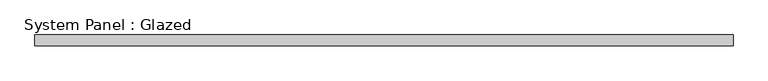
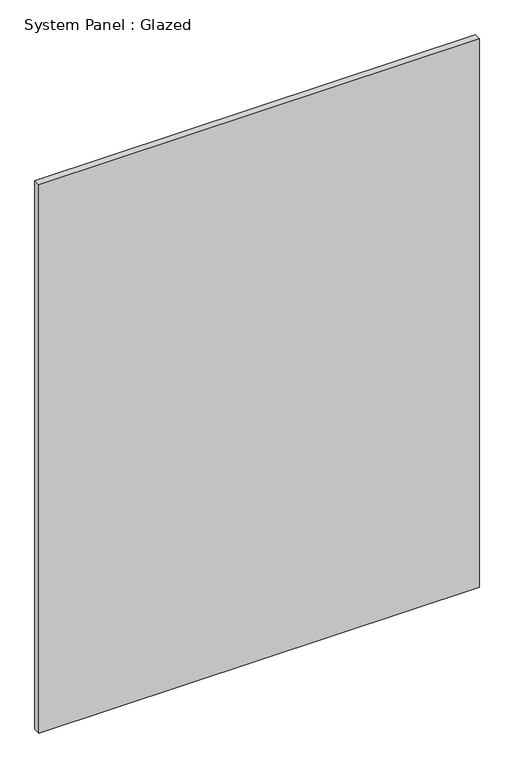
"""IFC4 building model written with IfcOpenShell, lengths in millimetres: plate geometry, System Panel : Glazed."""

import ifcopenshell
import ifcopenshell.guid

model = None  # the IFC model being written
_history = None  # IfcOwnerHistory: only IFC2X3 demands one
_inside = {}  # id of a spatial element -> (the spatial element, [elements in it])
_under = {}  # id of a project, library or spatial element -> (it, [spatial elements below it])
_declared = {}  # id of a project -> (the project, [libraries it declares])
_typed = {}  # id of a type object -> (the type object, [elements of that type])
_made_of = {}  # id of a material, layer set ... -> (it, [elements and type objects made of it])


def new_model(schema):
    """Start an empty IFC model of exactly this schema.

    Asked for "IFC4X3", IfcOpenShell would pick the latest addendum, in which some entities
    have other attributes; the version numbers below select the first issue.
    IFC2X3 requires an IfcOwnerHistory on every rooted entity: one is made here for all.
    """
    global model, _history
    if schema == "IFC4X3":
        model = ifcopenshell.file(schema_version=(4, 3, 0, 0))
    else:
        model = ifcopenshell.file(schema=schema)
    _inside.clear()
    _under.clear()
    _declared.clear()
    _typed.clear()
    _made_of.clear()
    _history = None
    if model.schema == "IFC2X3":
        org = make("IfcOrganization", Name="unknown")
        user = make(
            "IfcPersonAndOrganization",
            ThePerson=make("IfcPerson", FamilyName="unknown"),
            TheOrganization=org,
        )
        app = make(
            "IfcApplication",
            ApplicationDeveloper=org,
            Version="unknown",
            ApplicationFullName="unknown",
            ApplicationIdentifier="unknown",
        )
        _history = make(
            "IfcOwnerHistory",
            OwningUser=user,
            OwningApplication=app,
            ChangeAction="ADDED",
            CreationDate=0,
        )
    return model


def make(cls, **values):
    """One entity of the class cls with the attributes given. An attribute that is None is left unset."""
    return model.create_entity(
        cls, **{name: value for name, value in values.items() if value is not None}
    )


def rooted(cls, **values):
    """An entity with a GlobalId (a new one), such as an element, a storey or a relation."""
    return make(cls, GlobalId=ifcopenshell.guid.new(), OwnerHistory=_history, **values)


def si_unit(unit_type, name, prefix=None):
    """IfcSIUnit, for example si_unit("LENGTHUNIT", "METRE", prefix="MILLI")."""
    return make("IfcSIUnit", UnitType=unit_type, Prefix=prefix, Name=name)


def assignment(units):
    """IfcUnitAssignment: the units of a project."""
    return None if units is None else make("IfcUnitAssignment", Units=units)


def point(xyz):
    """IfcCartesianPoint."""
    return None if xyz is None else make("IfcCartesianPoint", Coordinates=xyz)


def direction(xyz):
    """IfcDirection."""
    return None if xyz is None else make("IfcDirection", DirectionRatios=xyz)


def frame(location, z_axis=None, x_axis=None):
    """IfcAxis2Placement3D, a coordinate frame: its origin and axes. An axis left out is left unset."""
    return make(
        "IfcAxis2Placement3D",
        Location=point(location),
        Axis=direction(z_axis),
        RefDirection=direction(x_axis),
    )


def origin():
    """The frame at (0, 0, 0) with its axes left unset."""
    return frame((0.0, 0.0, 0.0))


def origin_with_axes():
    """The frame at (0, 0, 0) with the z axis (0, 0, 1) and the x axis (1, 0, 0) written out."""
    return frame((0.0, 0.0, 0.0), z_axis=(0.0, 0.0, 1.0), x_axis=(1.0, 0.0, 0.0))


def place(relative_to, where):
    """IfcLocalPlacement: puts the frame where relative to a parent placement (None: the world)."""
    return make(
        "IfcLocalPlacement", PlacementRelTo=relative_to, RelativePlacement=where
    )


def context(
    kind, dimensions, precision=None, world=None, true_north=None, identifier=None
):
    """IfcGeometricRepresentationContext, for example the 3D "Model" context."""
    return make(
        "IfcGeometricRepresentationContext",
        ContextIdentifier=identifier,
        ContextType=kind,
        CoordinateSpaceDimension=dimensions,
        Precision=precision,
        WorldCoordinateSystem=world,
        TrueNorth=true_north,
    )


def project(units=None, contexts=None):
    """IfcProject with its units and contexts."""
    return rooted(
        "IfcProject",
        Name="project",
        RepresentationContexts=contexts,
        UnitsInContext=assignment(units),
    )


def spatial(cls, under=None, at=None, **own):
    """A site, building, storey or space (cls), placed at a placement, below another one or the project."""
    s = rooted(cls, ObjectPlacement=at, **own)
    if under is not None:
        _under.setdefault(under.id(), (under, []))[1].append(s)
    return s


def polyline(points):
    """IfcPolyline through the points."""
    return make("IfcPolyline", Points=[point(p) for p in points])


def outline(outer, holes=None, kind="AREA"):
    """IfcArbitraryClosedProfileDef: a profile drawn as a closed curve; with holes, ...WithVoids."""
    if holes is None:
        return make("IfcArbitraryClosedProfileDef", ProfileType=kind, OuterCurve=outer)
    return make(
        "IfcArbitraryProfileDefWithVoids",
        ProfileType=kind,
        OuterCurve=outer,
        InnerCurves=holes,
    )


def extrude(swept, where, along, depth):
    """IfcExtrudedAreaSolid: the profile swept, set in the frame where, extruded along a direction by depth."""
    return make(
        "IfcExtrudedAreaSolid",
        SweptArea=swept,
        Position=where,
        ExtrudedDirection=direction(along),
        Depth=depth,
    )


def shape(context_of_items, identifier, shape_type, items):
    """IfcShapeRepresentation: the items that make up one representation, for example the "Body"."""
    return make(
        "IfcShapeRepresentation",
        ContextOfItems=context_of_items,
        RepresentationIdentifier=identifier,
        RepresentationType=shape_type,
        Items=items,
    )


def source(mapping_origin, context_of_items, identifier, shape_type, items):
    """IfcRepresentationMap: a shape defined once, which mapped items show again and again."""
    return make(
        "IfcRepresentationMap",
        MappingOrigin=mapping_origin,
        MappedRepresentation=shape(context_of_items, identifier, shape_type, items),
    )


def transform(
    local_origin,
    x_axis=None,
    y_axis=None,
    z_axis=None,
    scale=None,
    scale2=None,
    scale3=None,
    uniform=True,
):
    """IfcCartesianTransformationOperator3D, or its non-uniform kind. x_axis, y_axis, z_axis: its Axis1, 2, 3."""
    if uniform:
        return make(
            "IfcCartesianTransformationOperator3D",
            Axis1=direction(x_axis),
            Axis2=direction(y_axis),
            LocalOrigin=point(local_origin),
            Scale=scale,
            Axis3=direction(z_axis),
        )
    return make(
        "IfcCartesianTransformationOperator3DnonUniform",
        Axis1=direction(x_axis),
        Axis2=direction(y_axis),
        LocalOrigin=point(local_origin),
        Scale=scale,
        Axis3=direction(z_axis),
        Scale2=scale2,
        Scale3=scale3,
    )


def mapped(mapping_source, mapping_target):
    """IfcMappedItem: shows the shape of a source again, moved by a transform."""
    return make(
        "IfcMappedItem", MappingSource=mapping_source, MappingTarget=mapping_target
    )


def made_of(thing, what):
    """Note that an element or type object is made of a material, layer set ...; save() writes the relation."""
    if what is not None:
        _made_of.setdefault(what.id(), (what, []))[1].append(thing)
    return thing


def element(
    cls,
    number,
    at=None,
    inside=None,
    cuts=None,
    type_object=None,
    material=None,
    context=None,
    identifier="Body",
    shape_type=None,
    held_by="IfcProductDefinitionShape",
    body=None,
    shapes=None,
    **own,
):
    """One element of the class cls, such as IfcWall. Its Tag is "e" and its number.

    at: its placement. inside: the storey or other place that contains it. cuts: it is an
    opening in that element (IfcRelVoidsElement). A single representation is given by context,
    identifier, shape_type and body (its items); several are given by shapes. held_by: the class
    of the entity that holds the representations. save() writes the other relations.
    """
    e = rooted(cls, Tag="e%d" % number, ObjectPlacement=at, **own)
    if body is not None:
        shapes = [shape(context, identifier, shape_type, body)]
    if shapes is not None:
        e.Representation = make(held_by, Representations=shapes)
    if inside is not None:
        _inside.setdefault(inside.id(), (inside, []))[1].append(e)
    if cuts is not None:
        rooted(
            "IfcRelVoidsElement", RelatingBuildingElement=cuts, RelatedOpeningElement=e
        )
    if type_object is not None:
        _typed.setdefault(type_object.id(), (type_object, []))[1].append(e)
    return made_of(e, material)


def aggregate(whole, parts):
    """IfcRelAggregates: a whole, such as a stair, and the parts it consists of."""
    return rooted("IfcRelAggregates", RelatingObject=whole, RelatedObjects=parts)


def save(model, path):
    """Write the relations noted so far, then the file.

    IfcRelAggregates (storeys below a building ...), IfcRelContainedInSpatialStructure (elements
    in a storey), IfcRelDefinesByType, IfcRelAssociatesMaterial and IfcRelDeclares: one each for
    every whole, place, type object, material and project.
    """
    for whole, parts in _under.values():
        aggregate(whole, parts)
    for where, things in _inside.values():
        rooted(
            "IfcRelContainedInSpatialStructure",
            RelatedElements=things,
            RelatingStructure=where,
        )
    for kind, things in _typed.values():
        rooted("IfcRelDefinesByType", RelatedObjects=things, RelatingType=kind)
    for what, things in _made_of.values():
        rooted("IfcRelAssociatesMaterial", RelatedObjects=things, RelatingMaterial=what)
    for by, libraries in _declared.values():
        rooted("IfcRelDeclares", RelatingContext=by, RelatedDefinitions=libraries)
    model.write(path)


def system_panel_glazed_2d900ec6(model_context):
    return source(origin(), model_context, "Body", "SweptSolid", [
        extrude(outline(polyline([(807.775, -49.5), (-807.775, -49.5), (-807.775, -24.5), (807.775, -24.5), (807.775, -49.5)])), origin_with_axes(), (0.0, 0.0, 1.0), 2125.0),
    ])


if __name__ == "__main__":
    model = new_model("IFC4")
    model_context = context("Model", 3, world=origin())
    ifc_project = project(units=[si_unit("LENGTHUNIT", "METRE", prefix="MILLI")], contexts=[model_context])
    site = spatial("IfcSite", under=ifc_project)
    building = spatial("IfcBuilding", under=site)
    placement = place(None, origin())
    system_panel_glazed_shape = system_panel_glazed_2d900ec6(model_context)
    element("IfcPlate", 1, ObjectType="System Panel : Glazed", at=placement, inside=building, context=model_context, shape_type="MappedRepresentation", body=[
        mapped(system_panel_glazed_shape, transform((0.0, 0.0, 0.0), x_axis=(1.0, 0.0, 0.0), y_axis=(0.0, 1.0, 0.0), z_axis=(0.0, 0.0, 1.0))),
    ])
    save(model, "model.ifc")

# Revit data of these elements
# Type "System Panel : Glazed"
#   Keynote = "H11"
#   Construction Type Id = "GSP4R"
#   Analytic Construction = "1/8 in Pilkington single glazing"
#   Visual Light Transmittance = 0.9
#   Solar Heat Gain Coefficient = 0.86
#   Heat Transfer Coefficient (U) = 6.7069 W/(m²·K)
# Element 1 (IfcPlate, "System Panel : Glazed")
#   Materials on its faces: "Glass"
# Materials
#   "Glass": class "Glass", colour RGB 0 128 192, transparency 0.9, Description = "Soda Lime Glass", Cost = 0
